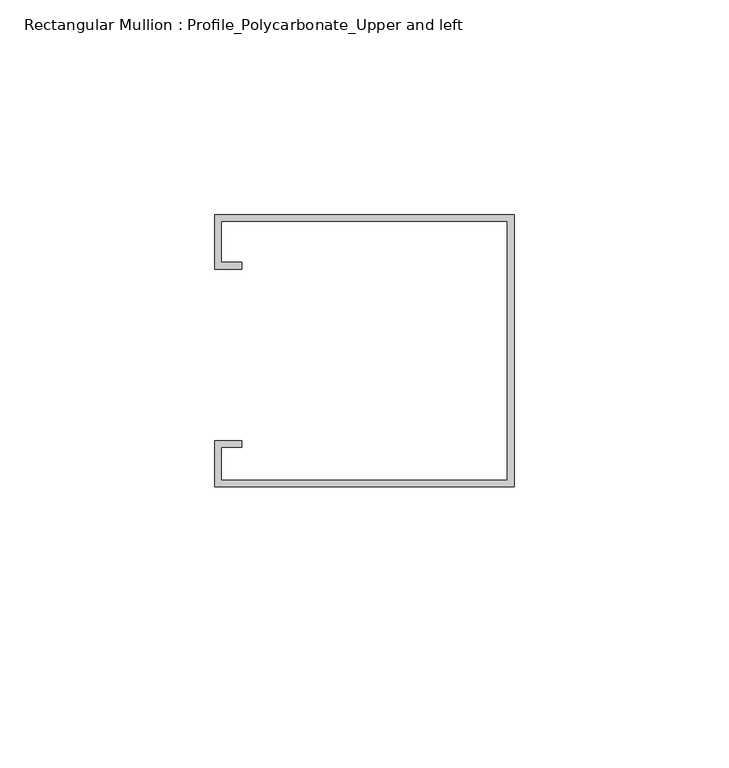
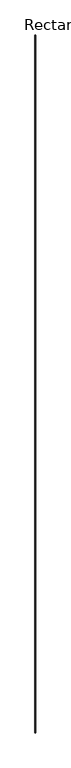
"""IFC4 building model written with IfcOpenShell, lengths in millimetres: member geometry, Rectangular Mullion : Profile_Polycarbonate_Upper and left."""

from ifc_helpers import new_model, si_unit, frame, origin, place, context, project, spatial, polyline, outline, extrude, source, transform, mapped, element, save


def rectangular_mullion_profile_polycarbonate_upper_and_left_92e5e834(model_context):
    return source(origin(), model_context, "Body", "SweptSolid", [
        extrude(outline(polyline([(0.0, 32.7), (0.0, -30.8), (-69.85, -30.8), (-69.85, -20.0), (-63.5, -20.0), (-63.5, -21.5875), (-68.2625, -21.5875), (-68.2625, -29.2125), (-1.5875, -29.2125), (-1.5875, 31.1125), (-68.2625, 31.1125), (-68.2625, 21.5875), (-63.5, 21.5875), (-63.5, 20.0), (-69.85, 20.0), (-69.85, 32.7), (0.0, 32.7)])), frame((0.0, 0.0, -88753.95), z_axis=(0.0, 0.0, 1.0), x_axis=(1.0, 0.0, 0.0)), (0.0, 0.0, 1.0), 88753.95),
    ])


if __name__ == "__main__":
    model = new_model("IFC4")
    model_context = context("Model", 3, world=origin())
    ifc_project = project(units=[si_unit("LENGTHUNIT", "METRE", prefix="MILLI")], contexts=[model_context])
    site = spatial("IfcSite", under=ifc_project)
    building = spatial("IfcBuilding", under=site)
    placement = place(None, origin())
    rectangular_mullion_profile_polycarbonate_upper_and_left_shape = rectangular_mullion_profile_polycarbonate_upper_and_left_92e5e834(model_context)
    element("IfcMember", 1, ObjectType="Rectangular Mullion : Profile_Polycarbonate_Upper and left", at=placement, inside=building, context=model_context, shape_type="MappedRepresentation", body=[
        mapped(rectangular_mullion_profile_polycarbonate_upper_and_left_shape, transform((0.0, 0.0, 0.0), x_axis=(1.0, 0.0, 0.0), y_axis=(0.0, 1.0, 0.0), z_axis=(0.0, 0.0, 1.0))),
    ])
    save(model, "model.ifc")

# Revit data of these elements
# Type "Rectangular Mullion : Profile_Polycarbonate_Upper and left"
#   built-in parameter 1007322 = 0.208333 (stored number, unit not read)
#   built-in parameter 1007321 = 0.00520833 (stored number, unit not read)
#   built-in parameter 1007320 = 0 (stored number, unit not read)
